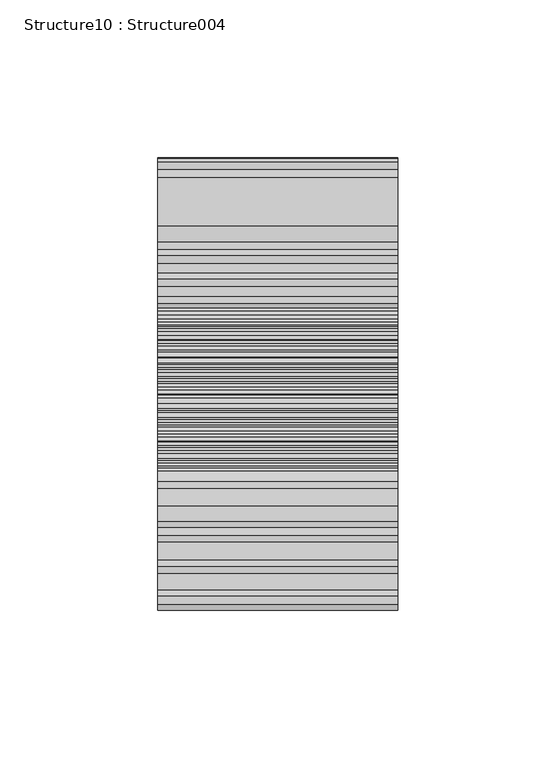
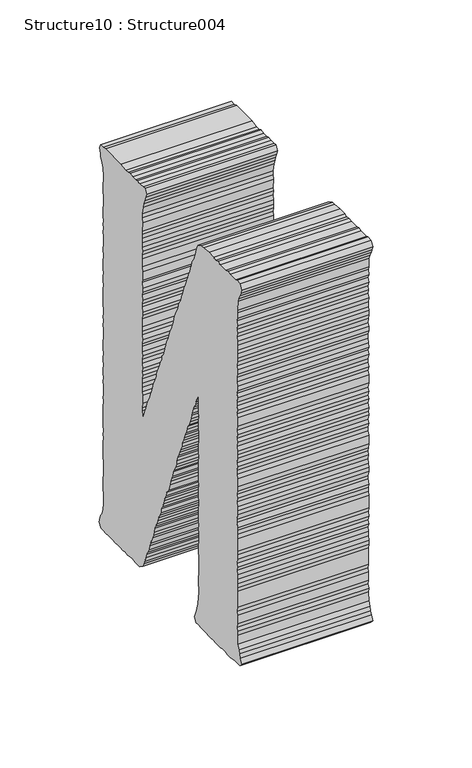
"""IFC4 building model written with IfcOpenShell, lengths in millimetres: proxy geometry, Structure10 : Structure004."""

from ifc_helpers import new_model, si_unit, frame, origin, place, context, project, spatial, polyline, outline, extrude, source, transform, mapped, element, save


def structure10_structure004_be604f00(model_context):
    return source(origin(), model_context, "Body", "SweptSolid", [
        extrude(outline(polyline([(4.3730473, 0.0), (7.5507006, 0.4771213), (9.447333, 0.52968), (14.6047587, 1.6773315), (17.1453244, -0.2503978), (16.4846309, -2.6527648), (16.4531781, -5.1432883), (15.7164154, -10.3515786), (15.7605694, -12.2350435), (15.3699393, -14.996469), (14.7639281, -17.0848603), (14.677793, -19.8893596), (14.0268218, -24.4911764), (13.1044698, -26.5476522), (12.6726645, -29.6001515), (13.0297182, -31.5398578), (12.6852469, -33.9749789), (11.3723834, -38.7920416), (10.6785758, -43.6966757), (8.2899903, -45.2248831), (5.7420265, -43.3192089), (3.6861522, -42.3986532), (1.6160177, -41.4760803), (-0.9598187, -39.8642172), (-6.1210947, -38.8132495), (-8.6141347, -38.7814407), (-10.6707293, -37.8599275), (-13.170615, -37.8160272), (-18.3680004, -37.0808072), (-20.477481, -36.4726684), (-22.9689784, -36.4299547), (-32.7673419, -35.0438822), (-35.2553488, -35.0127853), (-37.7173124, -34.6645169), (-40.117163, -34.0041794), (-42.8794274, -33.6134306), (-45.2799816, -32.9641166), (-47.8159767, -33.2359639), (-49.5806587, -32.3557446), (-52.4169547, -32.5851114), (-55.1213001, -31.8817002), (-57.3232664, -31.8910666), (-64.9775824, -30.8082901), (-67.3816272, -30.1473593), (-69.8251364, -29.8017015), (-71.7133807, -29.8554468), (-74.6884932, -28.8040004), (-76.5272067, -28.5438968), (-79.6822576, -28.7281727), (-82.125767, -28.3825148), (-84.2244779, -27.7647764), (-86.9446261, -27.0702528), (-89.4352846, -27.0276578), (-91.5363769, -26.4207056), (-93.7225404, -26.4211843), (-96.5251083, -26.3455898), (-101.4213541, -25.6529688), (-103.7916708, -24.6870767), (-106.2360191, -24.3413001), (-108.7711752, -24.6132661), (-110.826931, -23.6918716), (-113.9777879, -23.8767408), (-115.7761979, -23.3014828), (-118.2650437, -23.2702673), (-120.9398554, -22.2613014), (-123.7895725, -22.4887697), (-125.5316062, -21.6117542), (-128.3679021, -21.841121), (-130.432885, -20.9184212), (-133.587936, -21.1026971), (-138.4934089, -20.4087709), (-140.5357434, -19.489275), (-143.0818044, -19.7596983), (-145.4420552, -18.7952301), (-147.5944907, -18.4907474), (-150.7361205, -18.6769219), (-153.0963713, -17.7124536), (-155.0359587, -18.0686685), (-157.4358093, -17.408331), (-160.1408585, -16.7159433), (-162.9031229, -16.3251945), (-165.134623, -16.6401155), (-167.884305, -16.2511466), (-169.63976, -15.3722325), (-172.4449795, -15.2851398), (-174.9464077, -15.2521444), (-177.6952508, -14.8632942), (-179.4810784, -14.2898161), (-182.5562261, -13.854807), (-185.045072, -13.8235914), (-187.4070004, -12.8588858), (-189.906886, -12.8149856), (-191.9979124, -12.2094573), (-194.5422957, -12.480118), (-197.2137521, -11.4716267), (-199.1306912, -11.8310454), (-202.1537918, -11.0825432), (-204.0361642, -11.1371192), (-209.5901081, -10.6603374), (-211.8206507, -10.9745383), (-214.7878373, -12.1231432), (-216.7147566, -12.4563373), (-219.288555, -13.0317138), (-221.8062812, -10.8094615), (-221.7159518, -8.0055554), (-220.8382162, -6.2644792), (-220.099911, -1.0452842), (-220.417332, 1.174591), (-219.4934375, 3.2419717), (-218.7154997, 8.7413356), (-219.0297169, 10.9838592), (-218.0645286, 13.3431524), (-218.4231248, 15.2719537), (-217.7293172, 20.1765878), (-216.3307809, 25.5992852), (-216.0274849, 27.7433326), (-213.7116295, 30.8501704), (-211.7544727, 31.4999427), (-208.5911521, 31.6821931), (-206.3303556, 32.3009912), (-204.0576967, 32.9189669), (-202.1266161, 33.2755295), (-199.4672635, 34.4557019), (-196.5748285, 34.9851487), (-194.300492, 35.602887), (-192.0556894, 35.9150707), (-189.1355005, 36.7374897), (-187.2623552, 36.7933709), (-184.6307401, 37.6685901), (-182.0527475, 38.2433734), (-179.47989, 38.8060488), (-177.4623142, 39.7801084), (-175.2317716, 40.0943093), (-172.643713, 40.6676686), (-170.684895, 41.3291845), (-167.83528, 41.543833), (-165.477067, 42.7666044), (-163.2464057, 43.0816441), (-160.4010014, 43.3088669), (-157.7366158, 44.4883274), (-153.4933953, 45.7661576), (-151.2149833, 46.3824638), (-148.7294764, 46.3397419), (-146.1070883, 47.2162664), (-143.2196863, 47.7464251), (-140.9025135, 48.6669808), (-139.2776056, 49.0668545), (-136.0957581, 49.5433825), (-134.4691726, 49.9430189), (-131.8466822, 50.832363), (-128.9584414, 51.3624032), (-126.7312213, 51.6531168), (-124.4553423, 52.2817598), (-121.6166322, 52.497951), (-119.8605962, 53.8187404), (-117.3742504, 53.7758999), (-115.0151987, 54.9985528), (-112.1656002, 55.2251822), (-109.532205, 56.1129838), (-107.2697144, 56.7195636), (-104.9954966, 57.3364631), (-103.1139466, 57.3791768), (-99.8765945, 58.1815429), (-97.561218, 59.1014971), (-95.2886614, 59.706653), (-92.7393637, 59.9757629), (-90.2076815, 60.2473646), (-88.2479059, 60.9096006), (-85.6608048, 61.4822399), (-83.0409168, 62.3471393), (-81.0274165, 63.322631), (-76.2492374, 63.8941981), (-73.990941, 64.5013713), (-70.7528688, 65.3027798), (-68.4659498, 65.9187383), (-68.9968328, 66.6235693), (-71.3705906, 67.5651355), (-73.2000771, 67.8239339), (-76.3466539, 67.663272), (-81.2529657, 68.3573169), (-83.0076676, 69.2113117), (-85.7607049, 69.6007552), (-88.2453894, 69.6553394), (-91.0168809, 70.0473934), (-93.5082597, 70.0909458), (-95.2537345, 70.9436354), (-97.7955156, 70.6974193), (-100.1600463, 71.6376803), (-102.6178157, 71.9853553), (-105.4498317, 71.7801958), (-107.5510425, 72.3863093), (-110.5724326, 73.1106122), (-112.4573543, 73.0803542), (-114.9344729, 73.1218893), (-117.6227917, 74.1079532), (-120.1116704, 74.1631306), (-122.5148434, 74.7999808), (-127.4203163, 75.4939071), (-129.9612585, 75.2475724), (-131.7907449, 75.5063708), (-134.7600714, 76.5321859), (-136.6122063, 76.7941881), (-139.145599, 76.5467855), (-142.1653278, 77.2828321), (-144.0468778, 77.2401184), (-146.4819988, 77.5845896), (-149.4731349, 78.6134899), (-151.3874717, 78.2785159), (-156.2937835, 78.9725608), (-159.3135124, 79.7086074), (-164.2189852, 80.4025336), (-166.3084362, 80.9950048), (-168.8544113, 80.7493821), (-170.9547834, 81.3553769), (-173.7036266, 81.7442271), (-176.4339429, 82.4273549), (-178.9236605, 82.482651), (-180.7211988, 83.0338284), (-186.3020579, 83.2175191), (-188.6808487, 84.1597973), (-191.1235192, 84.5053365), (-195.8538452, 84.2478556), (-198.7370531, 83.7171036), (-200.9777802, 83.4034878), (-203.8987915, 82.5692064), (-206.4750042, 82.0070056), (-209.023103, 83.923822), (-208.4144731, 86.024677), (-207.9810065, 89.0889198), (-207.9403265, 91.5781381), (-207.0742322, 93.3336952), (-206.6408843, 96.3970993), (-206.9003865, 98.9296369), (-206.0342921, 100.685194), (-205.6882783, 103.1312199), (-205.6001054, 108.1215268), (-203.4345525, 123.430159), (-202.4811241, 125.8030944), (-202.4352924, 128.2924395), (-199.8465137, 128.8648413), (-196.9149577, 127.5115352), (-195.1148865, 126.9480209), (-192.5399913, 125.3234566), (-190.220797, 124.0687535), (-185.0998573, 122.7265936), (-183.2619826, 122.4666086), (-180.1087115, 122.6383019), (-175.520316, 121.9892294), (-173.1490583, 121.0360383), (-167.9516728, 120.3008183), (-166.0659287, 120.3429386), (-160.8467337, 119.6046334), (-158.4544491, 118.9573449), (-155.9672644, 118.9143856), (-153.8534711, 118.3064924), (-151.3662865, 118.2635331), (-148.6468585, 117.569967), (-143.7548068, 116.8779394), (-141.2063316, 117.1351869), (-136.3999527, 115.8375247), (-133.8573493, 116.0956029), (-131.1505038, 115.4038167), (-128.9947128, 115.0988594), (-126.2878672, 114.4070732), (-124.372708, 114.7539093), (-121.2958827, 114.3186629), (-119.2391858, 113.4099695), (-116.7520012, 113.3670103), (-111.5411945, 112.6298917), (-109.3459224, 112.6282263), (-106.6399157, 111.9365588), (-104.8532657, 111.3749431), (-102.3963351, 111.0273866), (-99.5996226, 110.9406417), (-97.4984116, 110.3345284), (-94.6983438, 110.2473088), (-91.9780769, 109.553624), (-87.0868641, 108.8617151), (-84.8571439, 109.1640536), (-79.951671, 108.4701274), (-77.8798752, 107.5592981), (-74.7878948, 107.4307847), (-72.915572, 107.4748036), (-70.5434754, 106.521494), (-68.0529355, 106.4780601), (-65.6043932, 106.1316903), (-62.5754372, 105.3943385), (-60.7031144, 105.4383574), (-57.6783526, 104.7015989), (-52.7770738, 104.0082659), (-50.5473536, 104.3106045), (-48.489818, 103.4017925), (-45.3793833, 103.2706685), (-42.8796162, 103.2259294), (-40.7926655, 102.6218333), (-33.1375105, 101.5389382), (-31.0237171, 100.9310449), (-28.2320376, 100.8450119), (-26.4311275, 100.281379), (-23.3257258, 100.150967), (-21.4534031, 100.1949859), (-18.4336742, 99.4589394), (-16.2333691, 99.456562), (-13.7898599, 99.1109042), (-11.7323241, 98.2020922), (-4.0771692, 97.1191971), (-1.2720684, 97.0312656), (0.9005553, 97.032804), (3.6342434, 96.3372207), (5.5065661, 96.3812396), (8.1781248, 95.3855681), (13.3889315, 94.6484495), (17.7618602, 94.6476106), (20.9395135, 95.1247319), (22.9664351, 96.0983251), (26.1507825, 96.586478), (28.0810243, 96.9431593), (30.5786349, 94.7117738), (30.2754575, 92.5685653), (30.2749952, 90.3697005), (29.5388135, 87.3611139), (29.2355174, 85.2170665), (28.5303263, 82.5001386), (28.8907025, 80.5839196), (28.1510797, 77.5510068), (27.8924, 75.7223592), (27.7634284, 72.6150425), (26.8394151, 70.546823), (27.1124573, 68.0132258), (26.1044324, 65.3511152), (25.8439727, 63.5098852), (26.1170149, 60.9762879), (25.4218897, 58.2579361), (25.1187123, 56.1147276), (22.5319713, 53.355086), (20.2678194, 52.7367626), (17.6066868, 51.5440078), (15.4063818, 51.546385), (12.5290294, 51.0267833), (10.1968926, 50.0972215), (7.8939799, 49.1746485), (5.0443814, 48.9480191), (2.4152662, 48.0844248), (-2.1316104, 46.8495496), (-4.3982624, 46.2196013), (-6.2915723, 46.1905298), (-9.4708868, 45.7016649), (-11.4440837, 45.0413275), (-14.1059364, 43.8495301), (-16.2919813, 43.8498902), (-18.9269518, 42.9751457), (-21.2004495, 42.3572887), (-23.5032437, 41.4355545), (-26.3192329, 41.5130477), (-28.320065, 40.5605769), (-30.9526212, 39.6726565), (-33.1302779, 39.6718301), (-35.7526495, 38.7833247), (-37.6753746, 38.4495373), (-40.2540874, 37.8757115), (-42.6241463, 36.6417815), (-47.4762381, 35.4509375), (-49.9634227, 35.4938967), (-52.5850905, 34.6164148), (-54.5673958, 33.9582214), (-57.708068, 33.7727672), (-59.37499, 33.0819384), (-61.9932862, 32.1920009), (-64.5854203, 31.6200737), (-66.772304, 31.6205525), (-69.6496564, 31.1009507), (-71.6185404, 30.4408588), (-74.2410307, 29.5515146), (-76.1670784, 29.19424), (-79.146025, 28.0592772), (-81.6365648, 28.102711), (-84.2674598, 27.2265344), (-86.4845811, 26.910435), (-89.1170187, 26.0233535), (-90.7302159, 25.6457804), (-93.967568, 24.8434143), (-96.1981106, 24.5292134), (-98.2417791, 23.2739253), (-100.5294181, 22.6589243), (-103.1048779, 22.0718042), (-105.6483202, 21.8138446), (-107.5651407, 21.4552647), (-110.4416542, 20.9355443), (-113.1220798, 19.7455186), (-115.3534613, 19.4314364), (-117.3223454, 18.7713445), (-119.898558, 18.2091437), (-122.529453, 17.332967), (-120.1161813, 16.670731), (-117.9368634, 16.6833012), (-114.8617157, 16.248292), (-112.762166, 15.630435), (-110.3606543, 14.9818412), (-108.1746094, 14.981481), (-103.2682976, 14.2874362), (-100.2485687, 13.5513896), (-95.9613129, 12.9449161), (-92.8517171, 12.8139109), (-90.977733, 12.8696734), (-88.5644613, 12.2074374), (-85.8584545, 11.5157699), (-83.3225781, 11.7867783), (-78.1168044, 11.0503717), (-75.7035326, 10.3881356), (-73.5158264, 10.3995192), (-70.8114809, 9.696108), (-68.6968487, 9.088096), (-66.1660053, 9.3598164), (-63.4121292, 8.9702542), (-61.3041912, 8.3512106), (-59.2130462, 7.7465211), (-56.7552768, 7.3988461), (-54.5692319, 7.398486), (-51.5058278, 6.965138), (-49.0136266, 6.9334479), (-46.6137761, 6.2731104), (-44.4999827, 5.6652171), (-41.9641064, 5.9362256), (-39.3025973, 4.9299971), (-34.4013185, 4.2366641), (-32.2144347, 4.2361854), (-27.3089619, 3.5422591), (-25.2085897, 2.9362644), (-14.7911704, 1.4626205), (-12.6185467, 1.4641589), (-9.7975245, 1.3859539), (-7.6677374, 1.084675), (-5.5984416, 0.1622208), (-3.1540935, -0.1835557), (0.0, 0.0), (4.3730473, 0.0)])), frame((-35624.0862846, 277381.8332963, 3999.8318725), z_axis=(1.0, 0.0, 1.354250045437766e-12), x_axis=(1.3435374844757662e-12, 0.14006512962532752, -0.9901422925332704)), (0.0, 0.0, 1.0), 76.2),
    ])


if __name__ == "__main__":
    model = new_model("IFC4")
    model_context = context("Model", 3, world=origin())
    ifc_project = project(units=[si_unit("LENGTHUNIT", "METRE", prefix="MILLI")], contexts=[model_context])
    site = spatial("IfcSite", under=ifc_project)
    building = spatial("IfcBuilding", under=site)
    placement = place(None, origin())
    structure10_structure004_shape = structure10_structure004_be604f00(model_context)
    element("IfcBuildingElementProxy", 1, Name="Structure10 : Structure004", ObjectType="Structure10 : Structure004", at=placement, inside=building, context=model_context, shape_type="MappedRepresentation", body=[
        mapped(structure10_structure004_shape, transform((0.0, 0.0, 0.0), x_axis=(1.0, 0.0, 0.0), y_axis=(0.0, 1.0, 0.0), z_axis=(0.0, 0.0, 1.0))),
    ])
    save(model, "model.ifc")

# Revit data of these elements
# Type "Structure10 : Structure004"
#   NameOverride = "Structure004"
# Element 1 (IfcBuildingElementProxy, "Structure10 : Structure004")
#   Materials on its faces: "BRUSHED ALUMINUM LETTERING"
# Materials
#   "BRUSHED ALUMINUM LETTERING": class "Unassigned", colour RGB 169 181 186, transparency 0, Cost = 0
